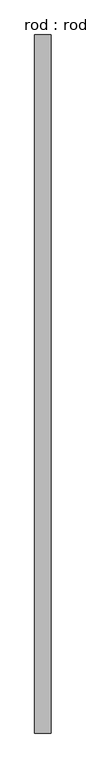
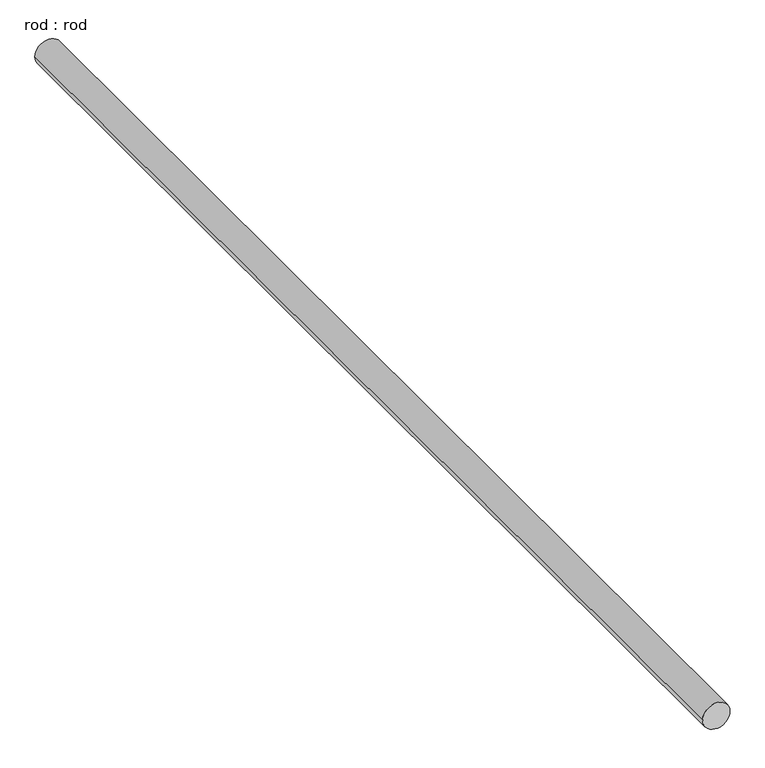
"""IFC4 building model written with IfcOpenShell, lengths in millimetres: proxy geometry, rod : rod."""

import ifcopenshell
import ifcopenshell.guid

model = None  # the IFC model being written
_history = None  # IfcOwnerHistory: only IFC2X3 demands one
_inside = {}  # id of a spatial element -> (the spatial element, [elements in it])
_under = {}  # id of a project, library or spatial element -> (it, [spatial elements below it])
_declared = {}  # id of a project -> (the project, [libraries it declares])
_typed = {}  # id of a type object -> (the type object, [elements of that type])
_made_of = {}  # id of a material, layer set ... -> (it, [elements and type objects made of it])


def new_model(schema):
    """Start an empty IFC model of exactly this schema.

    Asked for "IFC4X3", IfcOpenShell would pick the latest addendum, in which some entities
    have other attributes; the version numbers below select the first issue.
    IFC2X3 requires an IfcOwnerHistory on every rooted entity: one is made here for all.
    """
    global model, _history
    if schema == "IFC4X3":
        model = ifcopenshell.file(schema_version=(4, 3, 0, 0))
    else:
        model = ifcopenshell.file(schema=schema)
    _inside.clear()
    _under.clear()
    _declared.clear()
    _typed.clear()
    _made_of.clear()
    _history = None
    if model.schema == "IFC2X3":
        org = make("IfcOrganization", Name="unknown")
        user = make(
            "IfcPersonAndOrganization",
            ThePerson=make("IfcPerson", FamilyName="unknown"),
            TheOrganization=org,
        )
        app = make(
            "IfcApplication",
            ApplicationDeveloper=org,
            Version="unknown",
            ApplicationFullName="unknown",
            ApplicationIdentifier="unknown",
        )
        _history = make(
            "IfcOwnerHistory",
            OwningUser=user,
            OwningApplication=app,
            ChangeAction="ADDED",
            CreationDate=0,
        )
    return model


def make(cls, **values):
    """One entity of the class cls with the attributes given. An attribute that is None is left unset."""
    return model.create_entity(
        cls, **{name: value for name, value in values.items() if value is not None}
    )


def rooted(cls, **values):
    """An entity with a GlobalId (a new one), such as an element, a storey or a relation."""
    return make(cls, GlobalId=ifcopenshell.guid.new(), OwnerHistory=_history, **values)


def si_unit(unit_type, name, prefix=None):
    """IfcSIUnit, for example si_unit("LENGTHUNIT", "METRE", prefix="MILLI")."""
    return make("IfcSIUnit", UnitType=unit_type, Prefix=prefix, Name=name)


def assignment(units):
    """IfcUnitAssignment: the units of a project."""
    return None if units is None else make("IfcUnitAssignment", Units=units)


def point(xyz):
    """IfcCartesianPoint."""
    return None if xyz is None else make("IfcCartesianPoint", Coordinates=xyz)


def direction(xyz):
    """IfcDirection."""
    return None if xyz is None else make("IfcDirection", DirectionRatios=xyz)


def frame(location, z_axis=None, x_axis=None):
    """IfcAxis2Placement3D, a coordinate frame: its origin and axes. An axis left out is left unset."""
    return make(
        "IfcAxis2Placement3D",
        Location=point(location),
        Axis=direction(z_axis),
        RefDirection=direction(x_axis),
    )


def frame_2d(location, x_axis=None):
    """IfcAxis2Placement2D, a coordinate frame in the plane: its origin and x axis."""
    return make(
        "IfcAxis2Placement2D", Location=point(location), RefDirection=direction(x_axis)
    )


def origin():
    """The frame at (0, 0, 0) with its axes left unset."""
    return frame((0.0, 0.0, 0.0))


def place(relative_to, where):
    """IfcLocalPlacement: puts the frame where relative to a parent placement (None: the world)."""
    return make(
        "IfcLocalPlacement", PlacementRelTo=relative_to, RelativePlacement=where
    )


def context(
    kind, dimensions, precision=None, world=None, true_north=None, identifier=None
):
    """IfcGeometricRepresentationContext, for example the 3D "Model" context."""
    return make(
        "IfcGeometricRepresentationContext",
        ContextIdentifier=identifier,
        ContextType=kind,
        CoordinateSpaceDimension=dimensions,
        Precision=precision,
        WorldCoordinateSystem=world,
        TrueNorth=true_north,
    )


def project(units=None, contexts=None):
    """IfcProject with its units and contexts."""
    return rooted(
        "IfcProject",
        Name="project",
        RepresentationContexts=contexts,
        UnitsInContext=assignment(units),
    )


def spatial(cls, under=None, at=None, **own):
    """A site, building, storey or space (cls), placed at a placement, below another one or the project."""
    s = rooted(cls, ObjectPlacement=at, **own)
    if under is not None:
        _under.setdefault(under.id(), (under, []))[1].append(s)
    return s


def circle_curve(where, radius):
    """IfcCircle in the frame where."""
    return make("IfcCircle", Position=where, Radius=radius)


def trimmed(basis, trim1, trim2, sense, master):
    """IfcTrimmedCurve: the piece of a basis curve between two trims."""
    return make(
        "IfcTrimmedCurve",
        BasisCurve=basis,
        Trim1=trim1,
        Trim2=trim2,
        SenseAgreement=sense,
        MasterRepresentation=master,
    )


def segment(curve, same_sense, transition):
    """IfcCompositeCurveSegment."""
    return make(
        "IfcCompositeCurveSegment",
        Transition=transition,
        SameSense=same_sense,
        ParentCurve=curve,
    )


def composite_curve(segments, self_intersect=None):
    """IfcCompositeCurve: segments joined end to end."""
    return make("IfcCompositeCurve", Segments=segments, SelfIntersect=self_intersect)


def outline(outer, holes=None, kind="AREA"):
    """IfcArbitraryClosedProfileDef: a profile drawn as a closed curve; with holes, ...WithVoids."""
    if holes is None:
        return make("IfcArbitraryClosedProfileDef", ProfileType=kind, OuterCurve=outer)
    return make(
        "IfcArbitraryProfileDefWithVoids",
        ProfileType=kind,
        OuterCurve=outer,
        InnerCurves=holes,
    )


def extrude(swept, where, along, depth):
    """IfcExtrudedAreaSolid: the profile swept, set in the frame where, extruded along a direction by depth."""
    return make(
        "IfcExtrudedAreaSolid",
        SweptArea=swept,
        Position=where,
        ExtrudedDirection=direction(along),
        Depth=depth,
    )


def shape(context_of_items, identifier, shape_type, items):
    """IfcShapeRepresentation: the items that make up one representation, for example the "Body"."""
    return make(
        "IfcShapeRepresentation",
        ContextOfItems=context_of_items,
        RepresentationIdentifier=identifier,
        RepresentationType=shape_type,
        Items=items,
    )


def source(mapping_origin, context_of_items, identifier, shape_type, items):
    """IfcRepresentationMap: a shape defined once, which mapped items show again and again."""
    return make(
        "IfcRepresentationMap",
        MappingOrigin=mapping_origin,
        MappedRepresentation=shape(context_of_items, identifier, shape_type, items),
    )


def transform(
    local_origin,
    x_axis=None,
    y_axis=None,
    z_axis=None,
    scale=None,
    scale2=None,
    scale3=None,
    uniform=True,
):
    """IfcCartesianTransformationOperator3D, or its non-uniform kind. x_axis, y_axis, z_axis: its Axis1, 2, 3."""
    if uniform:
        return make(
            "IfcCartesianTransformationOperator3D",
            Axis1=direction(x_axis),
            Axis2=direction(y_axis),
            LocalOrigin=point(local_origin),
            Scale=scale,
            Axis3=direction(z_axis),
        )
    return make(
        "IfcCartesianTransformationOperator3DnonUniform",
        Axis1=direction(x_axis),
        Axis2=direction(y_axis),
        LocalOrigin=point(local_origin),
        Scale=scale,
        Axis3=direction(z_axis),
        Scale2=scale2,
        Scale3=scale3,
    )


def mapped(mapping_source, mapping_target):
    """IfcMappedItem: shows the shape of a source again, moved by a transform."""
    return make(
        "IfcMappedItem", MappingSource=mapping_source, MappingTarget=mapping_target
    )


def made_of(thing, what):
    """Note that an element or type object is made of a material, layer set ...; save() writes the relation."""
    if what is not None:
        _made_of.setdefault(what.id(), (what, []))[1].append(thing)
    return thing


def element(
    cls,
    number,
    at=None,
    inside=None,
    cuts=None,
    type_object=None,
    material=None,
    context=None,
    identifier="Body",
    shape_type=None,
    held_by="IfcProductDefinitionShape",
    body=None,
    shapes=None,
    **own,
):
    """One element of the class cls, such as IfcWall. Its Tag is "e" and its number.

    at: its placement. inside: the storey or other place that contains it. cuts: it is an
    opening in that element (IfcRelVoidsElement). A single representation is given by context,
    identifier, shape_type and body (its items); several are given by shapes. held_by: the class
    of the entity that holds the representations. save() writes the other relations.
    """
    e = rooted(cls, Tag="e%d" % number, ObjectPlacement=at, **own)
    if body is not None:
        shapes = [shape(context, identifier, shape_type, body)]
    if shapes is not None:
        e.Representation = make(held_by, Representations=shapes)
    if inside is not None:
        _inside.setdefault(inside.id(), (inside, []))[1].append(e)
    if cuts is not None:
        rooted(
            "IfcRelVoidsElement", RelatingBuildingElement=cuts, RelatedOpeningElement=e
        )
    if type_object is not None:
        _typed.setdefault(type_object.id(), (type_object, []))[1].append(e)
    return made_of(e, material)


def aggregate(whole, parts):
    """IfcRelAggregates: a whole, such as a stair, and the parts it consists of."""
    return rooted("IfcRelAggregates", RelatingObject=whole, RelatedObjects=parts)


def save(model, path):
    """Write the relations noted so far, then the file.

    IfcRelAggregates (storeys below a building ...), IfcRelContainedInSpatialStructure (elements
    in a storey), IfcRelDefinesByType, IfcRelAssociatesMaterial and IfcRelDeclares: one each for
    every whole, place, type object, material and project.
    """
    for whole, parts in _under.values():
        aggregate(whole, parts)
    for where, things in _inside.values():
        rooted(
            "IfcRelContainedInSpatialStructure",
            RelatedElements=things,
            RelatingStructure=where,
        )
    for kind, things in _typed.values():
        rooted("IfcRelDefinesByType", RelatedObjects=things, RelatingType=kind)
    for what, things in _made_of.values():
        rooted("IfcRelAssociatesMaterial", RelatedObjects=things, RelatingMaterial=what)
    for by, libraries in _declared.values():
        rooted("IfcRelDeclares", RelatingContext=by, RelatedDefinitions=libraries)
    model.write(path)


def rod_rod_fdba7ed2(model_context):
    return source(origin(), model_context, "Body", "SweptSolid", [
        extrude(outline(composite_curve([segment(trimmed(circle_curve(frame_2d((0.0108462, 0.0)), 200.0), [point((0.0108462, 200.0))], [point((0.0108462, -200.0))], False, "CARTESIAN"), True, "CONTINUOUS"), segment(trimmed(circle_curve(frame_2d((0.0108462, 0.0)), 200.0), [point((0.0108462, -200.0))], [point((0.0108462, 200.0))], False, "CARTESIAN"), True, "CONTINUOUS")], self_intersect=False)), frame((0.0, -4407.2713847, 0.0), z_axis=(0.0, 1.0, 0.0), x_axis=(0.0, 0.0, 1.0)), (0.0, 0.0, 1.0), 17000.0),
    ])


if __name__ == "__main__":
    model = new_model("IFC4")
    model_context = context("Model", 3, world=origin())
    ifc_project = project(units=[si_unit("LENGTHUNIT", "METRE", prefix="MILLI")], contexts=[model_context])
    site = spatial("IfcSite", under=ifc_project)
    building = spatial("IfcBuilding", under=site)
    placement = place(None, origin())
    rod_rod_shape = rod_rod_fdba7ed2(model_context)
    element("IfcBuildingElementProxy", 1, Name="rod : rod", ObjectType="rod : rod", at=placement, inside=building, context=model_context, shape_type="MappedRepresentation", body=[
        mapped(rod_rod_shape, transform((0.0, 0.0, 0.0), x_axis=(1.0, 0.0, 0.0), y_axis=(0.0, 1.0, 0.0), z_axis=(0.0, 0.0, 1.0))),
    ])
    save(model, "model.ifc")

# Revit data of these elements
# Type "rod : rod"
#   Default Elevation = 0
